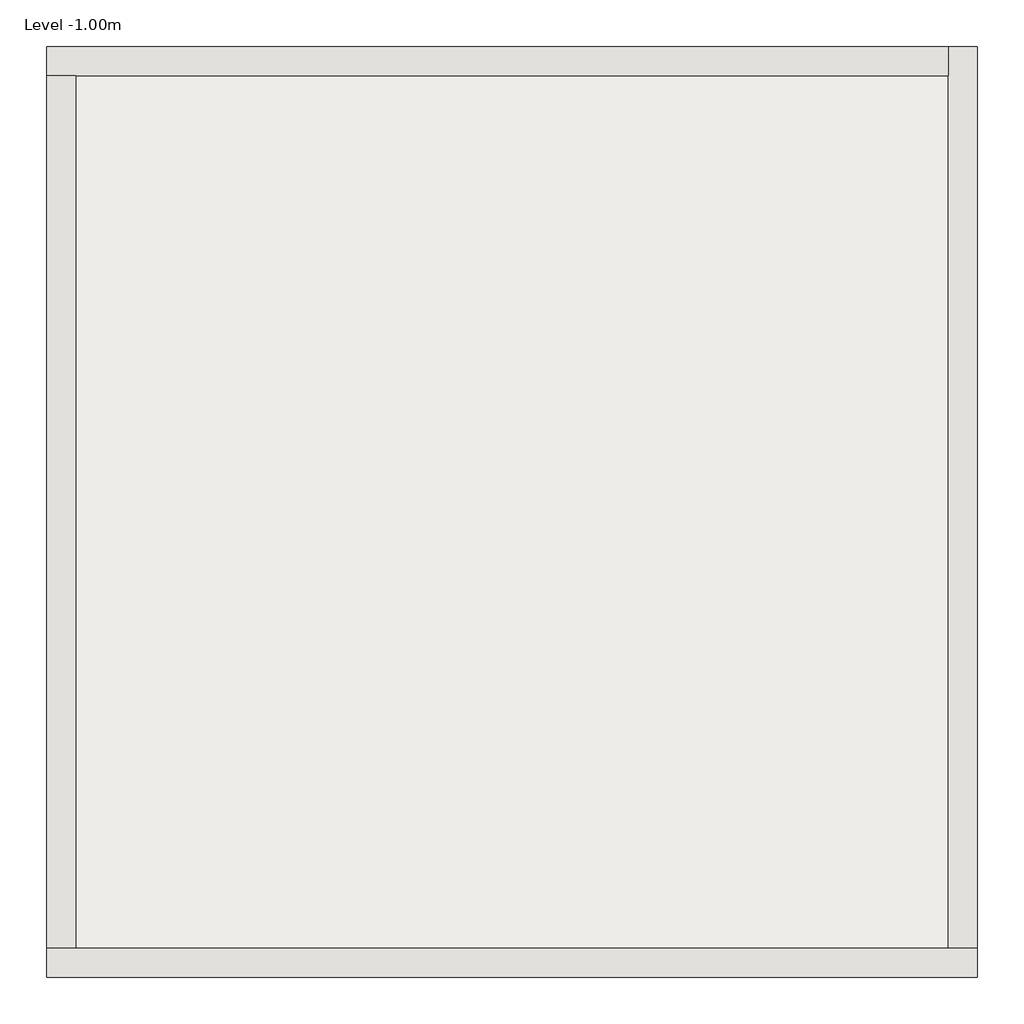
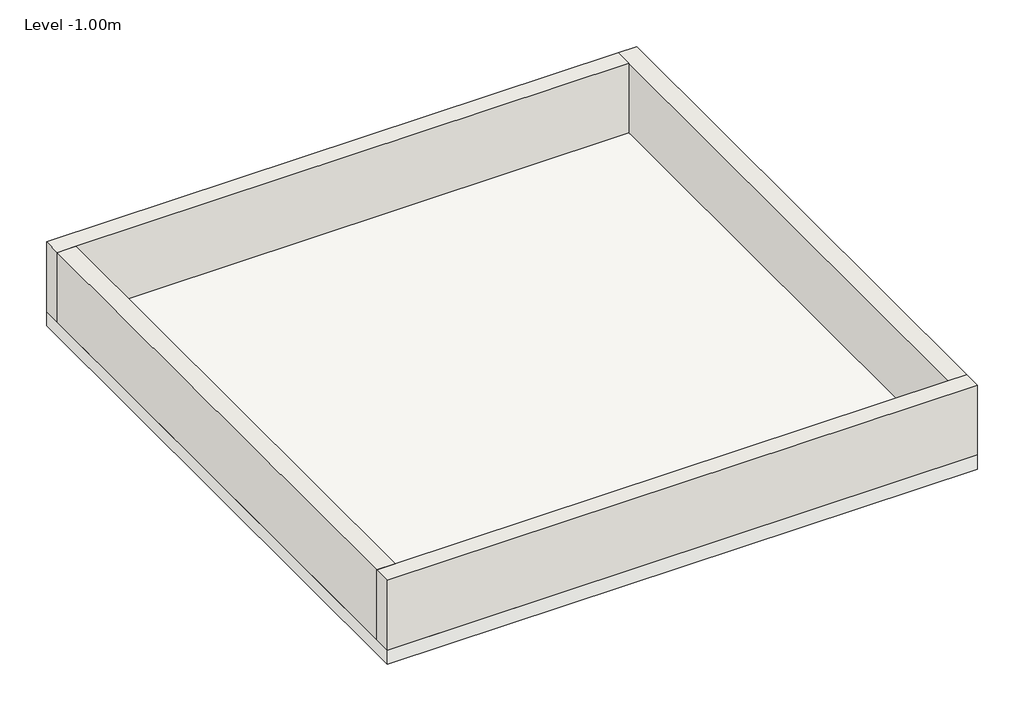
# One storey: 4 walls, 1 slab.
"""IFC4 building model written with IfcOpenShell, lengths in millimetres."""

from ifc_helpers import new_model, si_unit, frame, origin, place, context, project, spatial, polyline, outline, extrude, faceted_brep, element, save

model = new_model("IFC4")

# Units and contexts
model_context = context("Model", 3, world=origin())
ifc_project = project(units=[si_unit("LENGTHUNIT", "METRE", prefix="MILLI")], contexts=[model_context])

# Site, building, storey
site = spatial("IfcSite", under=ifc_project)
building = spatial("IfcBuilding", under=site)
storey = spatial("IfcBuildingStorey", under=building, Name="Level -1.00m", Elevation=-1000.000032)

# Slab
placement = place(None, origin())
element("IfcSlab", 1, ObjectType="SOL CAM SANIT", at=placement, inside=storey, context=model_context, shape_type="SweptSolid", body=[
    extrude(outline(polyline([(0.0, 7999.99416), (7999.99416, 7999.99416), (7999.99416, 0.0), (0.0, 0.0), (0.0, 7999.99416)])), frame((0.0, 0.0, -1203.0480384), z_axis=(0.0, 0.0, 1.0), x_axis=(1.0, 0.0, 0.0)), (0.0, 0.0, 1.0), 203.0480064),
])

# Walls
element("IfcWall", 2, ObjectType="MURO CAM SANIT", at=placement, inside=storey, context=model_context, shape_type="Brep", body=[
    faceted_brep([(0.0, 0.0, -1000.000032), (7999.99416, 0.0, -1000.000032), (7999.99416, 0.0, -0.012192), (0.0, 0.0, -0.012192), (0.0, 249.000008, -1000.000032), (0.0, 249.000008, -0.012192), (249.000008, 249.000008, -0.012192), (7750.994152, 249.000008, -0.012192), (7999.99416, 249.000008, -0.012192), (7999.99416, 249.000008, -1000.000032), (7750.994152, 249.000008, -1000.000032), (249.000008, 249.000008, -1000.000032)], [[[0, 1, 2, 3]], [[4, 5, 6, 7, 8, 9, 10, 11]], [[1, 0, 4, 11, 10, 9]], [[3, 2, 8, 7, 6, 5]], [[2, 1, 9, 8]], [[0, 3, 5, 4]]]),
])
element("IfcWall", 3, ObjectType="MURO CAM SANIT", at=placement, inside=storey, context=model_context, shape_type="Brep", body=[
    faceted_brep([(7999.99416, 249.000008, -1000.000032), (7999.99416, 7999.99416, -1000.000032), (7999.99416, 7999.99416, -0.012192), (7999.99416, 249.000008, -0.012192), (7750.994152, 249.000008, -1000.000032), (7750.994152, 249.000008, -0.012192), (7750.994152, 7750.994152, -0.012192), (7750.994152, 7999.99416, -0.012192), (7750.994152, 7999.99416, -1000.000032), (7750.994152, 7750.994152, -1000.000032)], [[[0, 1, 2, 3]], [[4, 5, 6, 7, 8, 9]], [[1, 0, 4, 9, 8]], [[3, 2, 7, 6, 5]], [[2, 1, 8, 7]], [[0, 3, 5, 4]]]),
])
element("IfcWall", 4, ObjectType="MURO CAM SANIT", at=placement, inside=storey, context=model_context, shape_type="Brep", body=[
    faceted_brep([(7750.994152, 7999.99416, -1000.000032), (0.0, 7999.99416, -1000.000032), (0.0, 7999.99416, -0.012192), (7750.994152, 7999.99416, -0.012192), (7750.994152, 7750.994152, -1000.000032), (7750.994152, 7750.994152, -0.012192), (249.000008, 7750.994152, -0.012192), (0.0, 7750.994152, -0.012192), (0.0, 7750.994152, -1000.000032), (249.000008, 7750.994152, -1000.000032)], [[[0, 1, 2, 3]], [[4, 5, 6, 7, 8, 9]], [[1, 0, 4, 9, 8]], [[3, 2, 7, 6, 5]], [[2, 1, 8, 7]], [[0, 3, 5, 4]]]),
])
element("IfcWall", 5, ObjectType="MURO CAM SANIT", at=placement, inside=storey, context=model_context, shape_type="SweptSolid", body=[
    extrude(outline(polyline([(0.0, 249.000008), (0.0, 7750.994152), (249.000008, 7750.994152), (249.000008, 249.000008), (0.0, 249.000008)])), frame((0.0, 0.0, -1000.000032), z_axis=(0.0, 0.0, 1.0), x_axis=(1.0, 0.0, 0.0)), (0.0, 0.0, 1.0), 999.98784),
])

save(model, "model.ifc")

# Revit data of these elements
# Project information
#   Organization Name = "Organization Name"
#   Organization Description = "Organization Description"
#   Building Name = "Building Name"
#   Project Issue Date = "Issue Date"
#   Project Status = "Project Status"
#   Client Name = "Client Name"
#   Project Address = "Enter address here\nAddress Line 2"
#   Project Name = "Project Name"
#   Project Number = "Project Number"
# Type "SOL CAM SANIT"
#   Layers, outside or top first: 80 mm no material (function 1); 3.048 mm no material (function 1); 120 mm no material (function 1)
# Type "MURO CAM SANIT"
#   Description = "Metal Studs with Brick over sheathing on exterior and Gypsum Wall Board (GWB) on interior, Exterior Function"
#   Assembly Code = "B2010158"
#   Type Mark = "W10"
#   Layers, outside or top first: 9 mm no material (function 1); 240 mm no material (function 1)
# Element 1 (IfcSlab, "SOL CAM SANIT")
#   Height Offset From Level = 0 mm
#   Phase Created = New Construction
# Elements 2, 3, 4, 5 (IfcWall, "MURO CAM SANIT")
#   Top Offset = 0 mm
#   Base Offset = 0 mm
#   Unconnected Height = 999.988 mm
#   wall height = 999.988 mm
#   Phase Created = New Construction
#   Base Constraint = Level -1.00m
#   Materials on its faces: "Default Wall"
# Materials
#   "Default Wall": class "Miscellaneous", colour RGB 192 192 192, transparency 0, Cost = 0
